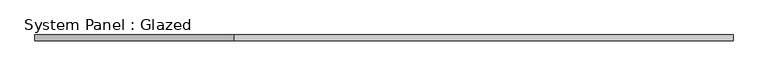
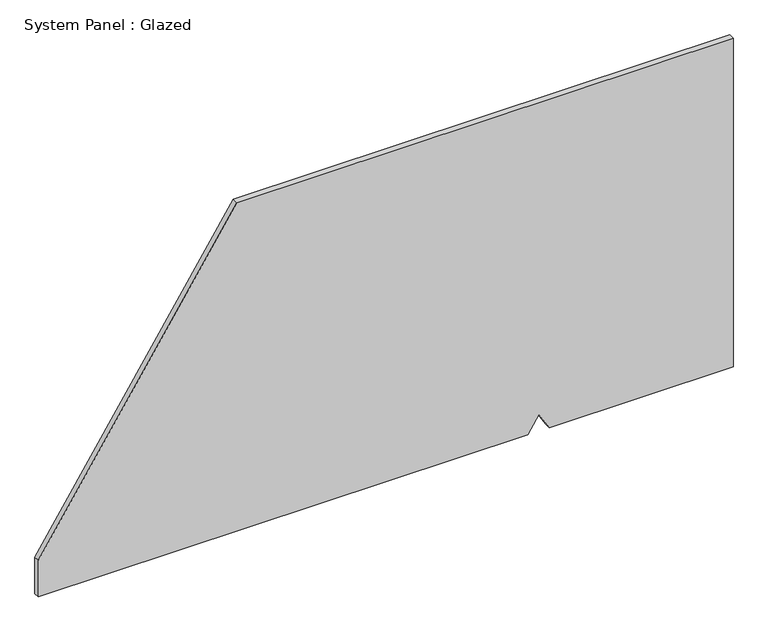
"""IFC4 building model written with IfcOpenShell, lengths in millimetres: plate geometry, System Panel : Glazed."""

import ifcopenshell
import ifcopenshell.guid

model = None  # the IFC model being written
_history = None  # IfcOwnerHistory: only IFC2X3 demands one
_inside = {}  # id of a spatial element -> (the spatial element, [elements in it])
_under = {}  # id of a project, library or spatial element -> (it, [spatial elements below it])
_declared = {}  # id of a project -> (the project, [libraries it declares])
_typed = {}  # id of a type object -> (the type object, [elements of that type])
_made_of = {}  # id of a material, layer set ... -> (it, [elements and type objects made of it])


def new_model(schema):
    """Start an empty IFC model of exactly this schema.

    Asked for "IFC4X3", IfcOpenShell would pick the latest addendum, in which some entities
    have other attributes; the version numbers below select the first issue.
    IFC2X3 requires an IfcOwnerHistory on every rooted entity: one is made here for all.
    """
    global model, _history
    if schema == "IFC4X3":
        model = ifcopenshell.file(schema_version=(4, 3, 0, 0))
    else:
        model = ifcopenshell.file(schema=schema)
    _inside.clear()
    _under.clear()
    _declared.clear()
    _typed.clear()
    _made_of.clear()
    _history = None
    if model.schema == "IFC2X3":
        org = make("IfcOrganization", Name="unknown")
        user = make(
            "IfcPersonAndOrganization",
            ThePerson=make("IfcPerson", FamilyName="unknown"),
            TheOrganization=org,
        )
        app = make(
            "IfcApplication",
            ApplicationDeveloper=org,
            Version="unknown",
            ApplicationFullName="unknown",
            ApplicationIdentifier="unknown",
        )
        _history = make(
            "IfcOwnerHistory",
            OwningUser=user,
            OwningApplication=app,
            ChangeAction="ADDED",
            CreationDate=0,
        )
    return model


def make(cls, **values):
    """One entity of the class cls with the attributes given. An attribute that is None is left unset."""
    return model.create_entity(
        cls, **{name: value for name, value in values.items() if value is not None}
    )


def rooted(cls, **values):
    """An entity with a GlobalId (a new one), such as an element, a storey or a relation."""
    return make(cls, GlobalId=ifcopenshell.guid.new(), OwnerHistory=_history, **values)


def si_unit(unit_type, name, prefix=None):
    """IfcSIUnit, for example si_unit("LENGTHUNIT", "METRE", prefix="MILLI")."""
    return make("IfcSIUnit", UnitType=unit_type, Prefix=prefix, Name=name)


def assignment(units):
    """IfcUnitAssignment: the units of a project."""
    return None if units is None else make("IfcUnitAssignment", Units=units)


def point(xyz):
    """IfcCartesianPoint."""
    return None if xyz is None else make("IfcCartesianPoint", Coordinates=xyz)


def direction(xyz):
    """IfcDirection."""
    return None if xyz is None else make("IfcDirection", DirectionRatios=xyz)


def frame(location, z_axis=None, x_axis=None):
    """IfcAxis2Placement3D, a coordinate frame: its origin and axes. An axis left out is left unset."""
    return make(
        "IfcAxis2Placement3D",
        Location=point(location),
        Axis=direction(z_axis),
        RefDirection=direction(x_axis),
    )


def origin():
    """The frame at (0, 0, 0) with its axes left unset."""
    return frame((0.0, 0.0, 0.0))


def place(relative_to, where):
    """IfcLocalPlacement: puts the frame where relative to a parent placement (None: the world)."""
    return make(
        "IfcLocalPlacement", PlacementRelTo=relative_to, RelativePlacement=where
    )


def context(
    kind, dimensions, precision=None, world=None, true_north=None, identifier=None
):
    """IfcGeometricRepresentationContext, for example the 3D "Model" context."""
    return make(
        "IfcGeometricRepresentationContext",
        ContextIdentifier=identifier,
        ContextType=kind,
        CoordinateSpaceDimension=dimensions,
        Precision=precision,
        WorldCoordinateSystem=world,
        TrueNorth=true_north,
    )


def project(units=None, contexts=None):
    """IfcProject with its units and contexts."""
    return rooted(
        "IfcProject",
        Name="project",
        RepresentationContexts=contexts,
        UnitsInContext=assignment(units),
    )


def spatial(cls, under=None, at=None, **own):
    """A site, building, storey or space (cls), placed at a placement, below another one or the project."""
    s = rooted(cls, ObjectPlacement=at, **own)
    if under is not None:
        _under.setdefault(under.id(), (under, []))[1].append(s)
    return s


def polyline(points):
    """IfcPolyline through the points."""
    return make("IfcPolyline", Points=[point(p) for p in points])


def outline(outer, holes=None, kind="AREA"):
    """IfcArbitraryClosedProfileDef: a profile drawn as a closed curve; with holes, ...WithVoids."""
    if holes is None:
        return make("IfcArbitraryClosedProfileDef", ProfileType=kind, OuterCurve=outer)
    return make(
        "IfcArbitraryProfileDefWithVoids",
        ProfileType=kind,
        OuterCurve=outer,
        InnerCurves=holes,
    )


def extrude(swept, where, along, depth):
    """IfcExtrudedAreaSolid: the profile swept, set in the frame where, extruded along a direction by depth."""
    return make(
        "IfcExtrudedAreaSolid",
        SweptArea=swept,
        Position=where,
        ExtrudedDirection=direction(along),
        Depth=depth,
    )


def shape(context_of_items, identifier, shape_type, items):
    """IfcShapeRepresentation: the items that make up one representation, for example the "Body"."""
    return make(
        "IfcShapeRepresentation",
        ContextOfItems=context_of_items,
        RepresentationIdentifier=identifier,
        RepresentationType=shape_type,
        Items=items,
    )


def source(mapping_origin, context_of_items, identifier, shape_type, items):
    """IfcRepresentationMap: a shape defined once, which mapped items show again and again."""
    return make(
        "IfcRepresentationMap",
        MappingOrigin=mapping_origin,
        MappedRepresentation=shape(context_of_items, identifier, shape_type, items),
    )


def transform(
    local_origin,
    x_axis=None,
    y_axis=None,
    z_axis=None,
    scale=None,
    scale2=None,
    scale3=None,
    uniform=True,
):
    """IfcCartesianTransformationOperator3D, or its non-uniform kind. x_axis, y_axis, z_axis: its Axis1, 2, 3."""
    if uniform:
        return make(
            "IfcCartesianTransformationOperator3D",
            Axis1=direction(x_axis),
            Axis2=direction(y_axis),
            LocalOrigin=point(local_origin),
            Scale=scale,
            Axis3=direction(z_axis),
        )
    return make(
        "IfcCartesianTransformationOperator3DnonUniform",
        Axis1=direction(x_axis),
        Axis2=direction(y_axis),
        LocalOrigin=point(local_origin),
        Scale=scale,
        Axis3=direction(z_axis),
        Scale2=scale2,
        Scale3=scale3,
    )


def mapped(mapping_source, mapping_target):
    """IfcMappedItem: shows the shape of a source again, moved by a transform."""
    return make(
        "IfcMappedItem", MappingSource=mapping_source, MappingTarget=mapping_target
    )


def made_of(thing, what):
    """Note that an element or type object is made of a material, layer set ...; save() writes the relation."""
    if what is not None:
        _made_of.setdefault(what.id(), (what, []))[1].append(thing)
    return thing


def element(
    cls,
    number,
    at=None,
    inside=None,
    cuts=None,
    type_object=None,
    material=None,
    context=None,
    identifier="Body",
    shape_type=None,
    held_by="IfcProductDefinitionShape",
    body=None,
    shapes=None,
    **own,
):
    """One element of the class cls, such as IfcWall. Its Tag is "e" and its number.

    at: its placement. inside: the storey or other place that contains it. cuts: it is an
    opening in that element (IfcRelVoidsElement). A single representation is given by context,
    identifier, shape_type and body (its items); several are given by shapes. held_by: the class
    of the entity that holds the representations. save() writes the other relations.
    """
    e = rooted(cls, Tag="e%d" % number, ObjectPlacement=at, **own)
    if body is not None:
        shapes = [shape(context, identifier, shape_type, body)]
    if shapes is not None:
        e.Representation = make(held_by, Representations=shapes)
    if inside is not None:
        _inside.setdefault(inside.id(), (inside, []))[1].append(e)
    if cuts is not None:
        rooted(
            "IfcRelVoidsElement", RelatingBuildingElement=cuts, RelatedOpeningElement=e
        )
    if type_object is not None:
        _typed.setdefault(type_object.id(), (type_object, []))[1].append(e)
    return made_of(e, material)


def aggregate(whole, parts):
    """IfcRelAggregates: a whole, such as a stair, and the parts it consists of."""
    return rooted("IfcRelAggregates", RelatingObject=whole, RelatedObjects=parts)


def save(model, path):
    """Write the relations noted so far, then the file.

    IfcRelAggregates (storeys below a building ...), IfcRelContainedInSpatialStructure (elements
    in a storey), IfcRelDefinesByType, IfcRelAssociatesMaterial and IfcRelDeclares: one each for
    every whole, place, type object, material and project.
    """
    for whole, parts in _under.values():
        aggregate(whole, parts)
    for where, things in _inside.values():
        rooted(
            "IfcRelContainedInSpatialStructure",
            RelatedElements=things,
            RelatingStructure=where,
        )
    for kind, things in _typed.values():
        rooted("IfcRelDefinesByType", RelatedObjects=things, RelatingType=kind)
    for what, things in _made_of.values():
        rooted("IfcRelAssociatesMaterial", RelatedObjects=things, RelatingMaterial=what)
    for by, libraries in _declared.values():
        rooted("IfcRelDeclares", RelatingContext=by, RelatedDefinitions=libraries)
    model.write(path)


def system_panel_glazed_56bc48d6(model_context):
    return source(origin(), model_context, "Body", "SweptSolid", [
        extrude(outline(polyline([(0.0, -1500.0), (0.0, 613.7086405), (75.6222799, 660.8350793), (0.0, 705.9127292), (0.0, 1500.0), (1500.0, 1500.0), (1500.0, -642.8120991), (166.61217, -1500.0), (0.0, -1500.0)])), frame((0.0, 24.5, 0.0), z_axis=(0.0, 1.0, 0.0), x_axis=(0.0, 0.0, 1.0)), (0.0, 0.0, 1.0), 25.0),
    ])


if __name__ == "__main__":
    model = new_model("IFC4")
    model_context = context("Model", 3, world=origin())
    ifc_project = project(units=[si_unit("LENGTHUNIT", "METRE", prefix="MILLI")], contexts=[model_context])
    site = spatial("IfcSite", under=ifc_project)
    building = spatial("IfcBuilding", under=site)
    placement = place(None, origin())
    system_panel_glazed_shape = system_panel_glazed_56bc48d6(model_context)
    element("IfcPlate", 1, ObjectType="System Panel : Glazed", at=placement, inside=building, context=model_context, shape_type="MappedRepresentation", body=[
        mapped(system_panel_glazed_shape, transform((0.0, 0.0, 0.0), x_axis=(1.0, 0.0, 0.0), y_axis=(0.0, 1.0, 0.0), z_axis=(0.0, 0.0, 1.0))),
    ])
    save(model, "model.ifc")

# Revit data of these elements
# Type "System Panel : Glazed"
#   Construction Type Id = "GSP4R"
#   Analytic Construction = "1/8 in Pilkington single glazing"
#   Visual Light Transmittance = 0.9
#   Solar Heat Gain Coefficient = 0.86
#   Heat Transfer Coefficient (U) = 6.7069 W/(m²·K)
#   Define Thermal Properties by = 1
# Element 1 (IfcPlate, "System Panel : Glazed")
#   Materials on its faces: "Glass"
# Materials
#   "Glass": class "Glass", colour RGB 0 128 192, transparency 0.9, Description = "Soda Lime Glass", Cost = 0
